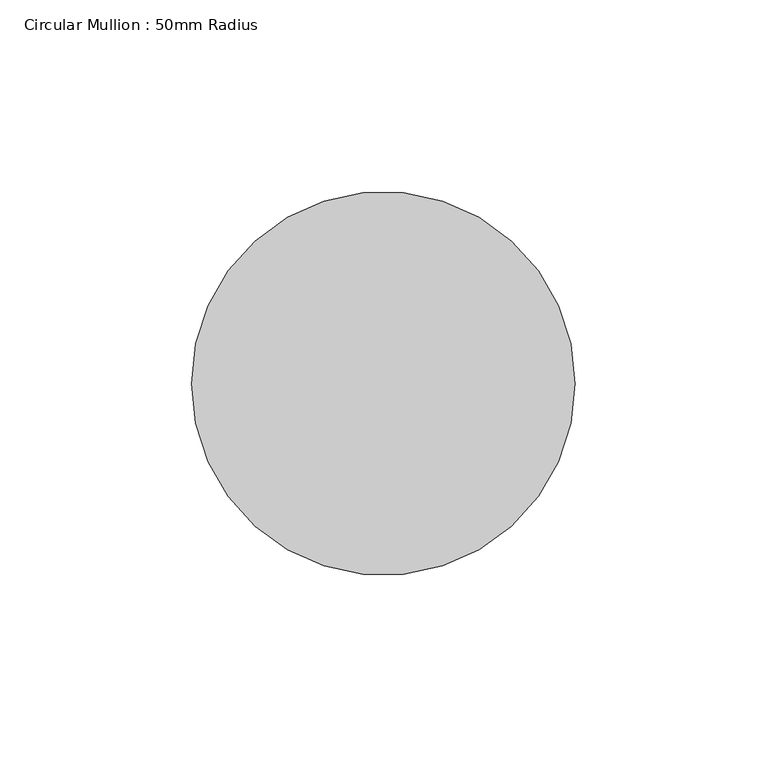
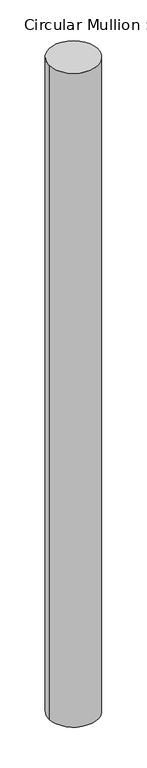
"""IFC4 building model written with IfcOpenShell, lengths in millimetres: member geometry, Circular Mullion : 50mm Radius."""

import ifcopenshell
import ifcopenshell.guid

model = None  # the IFC model being written
_history = None  # IfcOwnerHistory: only IFC2X3 demands one
_inside = {}  # id of a spatial element -> (the spatial element, [elements in it])
_under = {}  # id of a project, library or spatial element -> (it, [spatial elements below it])
_declared = {}  # id of a project -> (the project, [libraries it declares])
_typed = {}  # id of a type object -> (the type object, [elements of that type])
_made_of = {}  # id of a material, layer set ... -> (it, [elements and type objects made of it])


def new_model(schema):
    """Start an empty IFC model of exactly this schema.

    Asked for "IFC4X3", IfcOpenShell would pick the latest addendum, in which some entities
    have other attributes; the version numbers below select the first issue.
    IFC2X3 requires an IfcOwnerHistory on every rooted entity: one is made here for all.
    """
    global model, _history
    if schema == "IFC4X3":
        model = ifcopenshell.file(schema_version=(4, 3, 0, 0))
    else:
        model = ifcopenshell.file(schema=schema)
    _inside.clear()
    _under.clear()
    _declared.clear()
    _typed.clear()
    _made_of.clear()
    _history = None
    if model.schema == "IFC2X3":
        org = make("IfcOrganization", Name="unknown")
        user = make(
            "IfcPersonAndOrganization",
            ThePerson=make("IfcPerson", FamilyName="unknown"),
            TheOrganization=org,
        )
        app = make(
            "IfcApplication",
            ApplicationDeveloper=org,
            Version="unknown",
            ApplicationFullName="unknown",
            ApplicationIdentifier="unknown",
        )
        _history = make(
            "IfcOwnerHistory",
            OwningUser=user,
            OwningApplication=app,
            ChangeAction="ADDED",
            CreationDate=0,
        )
    return model


def make(cls, **values):
    """One entity of the class cls with the attributes given. An attribute that is None is left unset."""
    return model.create_entity(
        cls, **{name: value for name, value in values.items() if value is not None}
    )


def rooted(cls, **values):
    """An entity with a GlobalId (a new one), such as an element, a storey or a relation."""
    return make(cls, GlobalId=ifcopenshell.guid.new(), OwnerHistory=_history, **values)


def si_unit(unit_type, name, prefix=None):
    """IfcSIUnit, for example si_unit("LENGTHUNIT", "METRE", prefix="MILLI")."""
    return make("IfcSIUnit", UnitType=unit_type, Prefix=prefix, Name=name)


def assignment(units):
    """IfcUnitAssignment: the units of a project."""
    return None if units is None else make("IfcUnitAssignment", Units=units)


def point(xyz):
    """IfcCartesianPoint."""
    return None if xyz is None else make("IfcCartesianPoint", Coordinates=xyz)


def direction(xyz):
    """IfcDirection."""
    return None if xyz is None else make("IfcDirection", DirectionRatios=xyz)


def frame(location, z_axis=None, x_axis=None):
    """IfcAxis2Placement3D, a coordinate frame: its origin and axes. An axis left out is left unset."""
    return make(
        "IfcAxis2Placement3D",
        Location=point(location),
        Axis=direction(z_axis),
        RefDirection=direction(x_axis),
    )


def frame_2d(location, x_axis=None):
    """IfcAxis2Placement2D, a coordinate frame in the plane: its origin and x axis."""
    return make(
        "IfcAxis2Placement2D", Location=point(location), RefDirection=direction(x_axis)
    )


def origin():
    """The frame at (0, 0, 0) with its axes left unset."""
    return frame((0.0, 0.0, 0.0))


def origin_2d():
    """The frame at (0, 0) in the plane with its x axis left unset."""
    return frame_2d((0.0, 0.0))


def place(relative_to, where):
    """IfcLocalPlacement: puts the frame where relative to a parent placement (None: the world)."""
    return make(
        "IfcLocalPlacement", PlacementRelTo=relative_to, RelativePlacement=where
    )


def context(
    kind, dimensions, precision=None, world=None, true_north=None, identifier=None
):
    """IfcGeometricRepresentationContext, for example the 3D "Model" context."""
    return make(
        "IfcGeometricRepresentationContext",
        ContextIdentifier=identifier,
        ContextType=kind,
        CoordinateSpaceDimension=dimensions,
        Precision=precision,
        WorldCoordinateSystem=world,
        TrueNorth=true_north,
    )


def project(units=None, contexts=None):
    """IfcProject with its units and contexts."""
    return rooted(
        "IfcProject",
        Name="project",
        RepresentationContexts=contexts,
        UnitsInContext=assignment(units),
    )


def spatial(cls, under=None, at=None, **own):
    """A site, building, storey or space (cls), placed at a placement, below another one or the project."""
    s = rooted(cls, ObjectPlacement=at, **own)
    if under is not None:
        _under.setdefault(under.id(), (under, []))[1].append(s)
    return s


def circle_curve(where, radius):
    """IfcCircle in the frame where."""
    return make("IfcCircle", Position=where, Radius=radius)


def trimmed(basis, trim1, trim2, sense, master):
    """IfcTrimmedCurve: the piece of a basis curve between two trims."""
    return make(
        "IfcTrimmedCurve",
        BasisCurve=basis,
        Trim1=trim1,
        Trim2=trim2,
        SenseAgreement=sense,
        MasterRepresentation=master,
    )


def segment(curve, same_sense, transition):
    """IfcCompositeCurveSegment."""
    return make(
        "IfcCompositeCurveSegment",
        Transition=transition,
        SameSense=same_sense,
        ParentCurve=curve,
    )


def composite_curve(segments, self_intersect=None):
    """IfcCompositeCurve: segments joined end to end."""
    return make("IfcCompositeCurve", Segments=segments, SelfIntersect=self_intersect)


def outline(outer, holes=None, kind="AREA"):
    """IfcArbitraryClosedProfileDef: a profile drawn as a closed curve; with holes, ...WithVoids."""
    if holes is None:
        return make("IfcArbitraryClosedProfileDef", ProfileType=kind, OuterCurve=outer)
    return make(
        "IfcArbitraryProfileDefWithVoids",
        ProfileType=kind,
        OuterCurve=outer,
        InnerCurves=holes,
    )


def extrude(swept, where, along, depth):
    """IfcExtrudedAreaSolid: the profile swept, set in the frame where, extruded along a direction by depth."""
    return make(
        "IfcExtrudedAreaSolid",
        SweptArea=swept,
        Position=where,
        ExtrudedDirection=direction(along),
        Depth=depth,
    )


def shape(context_of_items, identifier, shape_type, items):
    """IfcShapeRepresentation: the items that make up one representation, for example the "Body"."""
    return make(
        "IfcShapeRepresentation",
        ContextOfItems=context_of_items,
        RepresentationIdentifier=identifier,
        RepresentationType=shape_type,
        Items=items,
    )


def source(mapping_origin, context_of_items, identifier, shape_type, items):
    """IfcRepresentationMap: a shape defined once, which mapped items show again and again."""
    return make(
        "IfcRepresentationMap",
        MappingOrigin=mapping_origin,
        MappedRepresentation=shape(context_of_items, identifier, shape_type, items),
    )


def transform(
    local_origin,
    x_axis=None,
    y_axis=None,
    z_axis=None,
    scale=None,
    scale2=None,
    scale3=None,
    uniform=True,
):
    """IfcCartesianTransformationOperator3D, or its non-uniform kind. x_axis, y_axis, z_axis: its Axis1, 2, 3."""
    if uniform:
        return make(
            "IfcCartesianTransformationOperator3D",
            Axis1=direction(x_axis),
            Axis2=direction(y_axis),
            LocalOrigin=point(local_origin),
            Scale=scale,
            Axis3=direction(z_axis),
        )
    return make(
        "IfcCartesianTransformationOperator3DnonUniform",
        Axis1=direction(x_axis),
        Axis2=direction(y_axis),
        LocalOrigin=point(local_origin),
        Scale=scale,
        Axis3=direction(z_axis),
        Scale2=scale2,
        Scale3=scale3,
    )


def mapped(mapping_source, mapping_target):
    """IfcMappedItem: shows the shape of a source again, moved by a transform."""
    return make(
        "IfcMappedItem", MappingSource=mapping_source, MappingTarget=mapping_target
    )


def made_of(thing, what):
    """Note that an element or type object is made of a material, layer set ...; save() writes the relation."""
    if what is not None:
        _made_of.setdefault(what.id(), (what, []))[1].append(thing)
    return thing


def element(
    cls,
    number,
    at=None,
    inside=None,
    cuts=None,
    type_object=None,
    material=None,
    context=None,
    identifier="Body",
    shape_type=None,
    held_by="IfcProductDefinitionShape",
    body=None,
    shapes=None,
    **own,
):
    """One element of the class cls, such as IfcWall. Its Tag is "e" and its number.

    at: its placement. inside: the storey or other place that contains it. cuts: it is an
    opening in that element (IfcRelVoidsElement). A single representation is given by context,
    identifier, shape_type and body (its items); several are given by shapes. held_by: the class
    of the entity that holds the representations. save() writes the other relations.
    """
    e = rooted(cls, Tag="e%d" % number, ObjectPlacement=at, **own)
    if body is not None:
        shapes = [shape(context, identifier, shape_type, body)]
    if shapes is not None:
        e.Representation = make(held_by, Representations=shapes)
    if inside is not None:
        _inside.setdefault(inside.id(), (inside, []))[1].append(e)
    if cuts is not None:
        rooted(
            "IfcRelVoidsElement", RelatingBuildingElement=cuts, RelatedOpeningElement=e
        )
    if type_object is not None:
        _typed.setdefault(type_object.id(), (type_object, []))[1].append(e)
    return made_of(e, material)


def aggregate(whole, parts):
    """IfcRelAggregates: a whole, such as a stair, and the parts it consists of."""
    return rooted("IfcRelAggregates", RelatingObject=whole, RelatedObjects=parts)


def save(model, path):
    """Write the relations noted so far, then the file.

    IfcRelAggregates (storeys below a building ...), IfcRelContainedInSpatialStructure (elements
    in a storey), IfcRelDefinesByType, IfcRelAssociatesMaterial and IfcRelDeclares: one each for
    every whole, place, type object, material and project.
    """
    for whole, parts in _under.values():
        aggregate(whole, parts)
    for where, things in _inside.values():
        rooted(
            "IfcRelContainedInSpatialStructure",
            RelatedElements=things,
            RelatingStructure=where,
        )
    for kind, things in _typed.values():
        rooted("IfcRelDefinesByType", RelatedObjects=things, RelatingType=kind)
    for what, things in _made_of.values():
        rooted("IfcRelAssociatesMaterial", RelatedObjects=things, RelatingMaterial=what)
    for by, libraries in _declared.values():
        rooted("IfcRelDeclares", RelatingContext=by, RelatedDefinitions=libraries)
    model.write(path)


def circular_mullion_50mm_radius_2efb4dff(model_context):
    return source(origin(), model_context, "Body", "SweptSolid", [
        extrude(outline(composite_curve([segment(trimmed(circle_curve(origin_2d(), 50.0), [point((50.0, 0.0))], [point((-50.0, 0.0))], False, "CARTESIAN"), True, "CONTINUOUS"), segment(trimmed(circle_curve(origin_2d(), 50.0), [point((-50.0, 0.0))], [point((50.0, 0.0))], False, "CARTESIAN"), True, "CONTINUOUS")], self_intersect=False)), frame((0.0, 0.0, -1407.7431683), z_axis=(0.0, 0.0, 1.0), x_axis=(1.0, 0.0, 0.0)), (0.0, 0.0, 1.0), 1407.7431683),
    ])


if __name__ == "__main__":
    model = new_model("IFC4")
    model_context = context("Model", 3, world=origin())
    ifc_project = project(units=[si_unit("LENGTHUNIT", "METRE", prefix="MILLI")], contexts=[model_context])
    site = spatial("IfcSite", under=ifc_project)
    building = spatial("IfcBuilding", under=site)
    placement = place(None, origin())
    circular_mullion_50mm_radius_shape = circular_mullion_50mm_radius_2efb4dff(model_context)
    element("IfcMember", 1, ObjectType="Circular Mullion : 50mm Radius", at=placement, inside=building, context=model_context, shape_type="MappedRepresentation", body=[
        mapped(circular_mullion_50mm_radius_shape, transform((0.0, 0.0, 0.0), x_axis=(1.0, 0.0, 0.0), y_axis=(0.0, 1.0, 0.0), z_axis=(0.0, 0.0, 1.0))),
    ])
    save(model, "model.ifc")

# Revit data of these elements
# Type "Circular Mullion : 50mm Radius"
#   built-in parameter 1007350 = 0.164042 (stored number, unit not read)
# Element 1 (IfcMember, "Circular Mullion : 50mm Radius")
#   Materials on its faces: "Aluminium"
# Materials
#   "Aluminium": class "Metal", colour RGB 247 247 247, transparency 0, Description = "Aluminium 6061", Cost = 0
